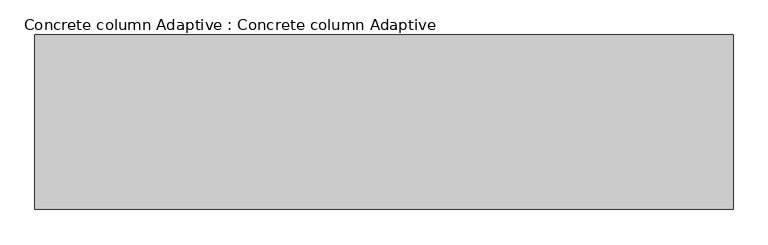
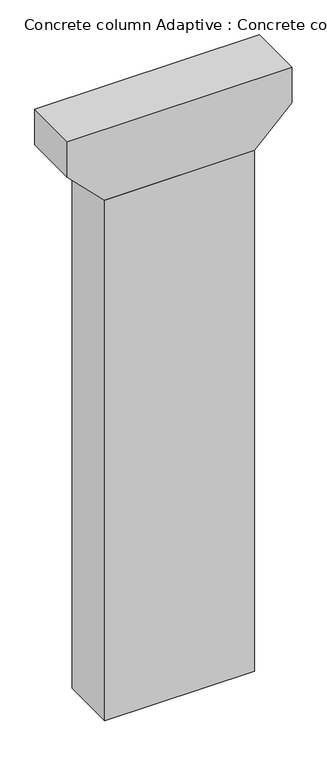
"""IFC4 building model written with IfcOpenShell, lengths in millimetres: proxy geometry, Concrete column Adaptive : Concrete column Adaptive."""

import ifcopenshell
import ifcopenshell.guid

model = None  # the IFC model being written
_history = None  # IfcOwnerHistory: only IFC2X3 demands one
_inside = {}  # id of a spatial element -> (the spatial element, [elements in it])
_under = {}  # id of a project, library or spatial element -> (it, [spatial elements below it])
_declared = {}  # id of a project -> (the project, [libraries it declares])
_typed = {}  # id of a type object -> (the type object, [elements of that type])
_made_of = {}  # id of a material, layer set ... -> (it, [elements and type objects made of it])


def new_model(schema):
    """Start an empty IFC model of exactly this schema.

    Asked for "IFC4X3", IfcOpenShell would pick the latest addendum, in which some entities
    have other attributes; the version numbers below select the first issue.
    IFC2X3 requires an IfcOwnerHistory on every rooted entity: one is made here for all.
    """
    global model, _history
    if schema == "IFC4X3":
        model = ifcopenshell.file(schema_version=(4, 3, 0, 0))
    else:
        model = ifcopenshell.file(schema=schema)
    _inside.clear()
    _under.clear()
    _declared.clear()
    _typed.clear()
    _made_of.clear()
    _history = None
    if model.schema == "IFC2X3":
        org = make("IfcOrganization", Name="unknown")
        user = make(
            "IfcPersonAndOrganization",
            ThePerson=make("IfcPerson", FamilyName="unknown"),
            TheOrganization=org,
        )
        app = make(
            "IfcApplication",
            ApplicationDeveloper=org,
            Version="unknown",
            ApplicationFullName="unknown",
            ApplicationIdentifier="unknown",
        )
        _history = make(
            "IfcOwnerHistory",
            OwningUser=user,
            OwningApplication=app,
            ChangeAction="ADDED",
            CreationDate=0,
        )
    return model


def make(cls, **values):
    """One entity of the class cls with the attributes given. An attribute that is None is left unset."""
    return model.create_entity(
        cls, **{name: value for name, value in values.items() if value is not None}
    )


def rooted(cls, **values):
    """An entity with a GlobalId (a new one), such as an element, a storey or a relation."""
    return make(cls, GlobalId=ifcopenshell.guid.new(), OwnerHistory=_history, **values)


def si_unit(unit_type, name, prefix=None):
    """IfcSIUnit, for example si_unit("LENGTHUNIT", "METRE", prefix="MILLI")."""
    return make("IfcSIUnit", UnitType=unit_type, Prefix=prefix, Name=name)


def assignment(units):
    """IfcUnitAssignment: the units of a project."""
    return None if units is None else make("IfcUnitAssignment", Units=units)


def point(xyz):
    """IfcCartesianPoint."""
    return None if xyz is None else make("IfcCartesianPoint", Coordinates=xyz)


def direction(xyz):
    """IfcDirection."""
    return None if xyz is None else make("IfcDirection", DirectionRatios=xyz)


def frame(location, z_axis=None, x_axis=None):
    """IfcAxis2Placement3D, a coordinate frame: its origin and axes. An axis left out is left unset."""
    return make(
        "IfcAxis2Placement3D",
        Location=point(location),
        Axis=direction(z_axis),
        RefDirection=direction(x_axis),
    )


def origin():
    """The frame at (0, 0, 0) with its axes left unset."""
    return frame((0.0, 0.0, 0.0))


def origin_with_axes():
    """The frame at (0, 0, 0) with the z axis (0, 0, 1) and the x axis (1, 0, 0) written out."""
    return frame((0.0, 0.0, 0.0), z_axis=(0.0, 0.0, 1.0), x_axis=(1.0, 0.0, 0.0))


def place(relative_to, where):
    """IfcLocalPlacement: puts the frame where relative to a parent placement (None: the world)."""
    return make(
        "IfcLocalPlacement", PlacementRelTo=relative_to, RelativePlacement=where
    )


def context(
    kind, dimensions, precision=None, world=None, true_north=None, identifier=None
):
    """IfcGeometricRepresentationContext, for example the 3D "Model" context."""
    return make(
        "IfcGeometricRepresentationContext",
        ContextIdentifier=identifier,
        ContextType=kind,
        CoordinateSpaceDimension=dimensions,
        Precision=precision,
        WorldCoordinateSystem=world,
        TrueNorth=true_north,
    )


def project(units=None, contexts=None):
    """IfcProject with its units and contexts."""
    return rooted(
        "IfcProject",
        Name="project",
        RepresentationContexts=contexts,
        UnitsInContext=assignment(units),
    )


def spatial(cls, under=None, at=None, **own):
    """A site, building, storey or space (cls), placed at a placement, below another one or the project."""
    s = rooted(cls, ObjectPlacement=at, **own)
    if under is not None:
        _under.setdefault(under.id(), (under, []))[1].append(s)
    return s


def polyline(points):
    """IfcPolyline through the points."""
    return make("IfcPolyline", Points=[point(p) for p in points])


def outline(outer, holes=None, kind="AREA"):
    """IfcArbitraryClosedProfileDef: a profile drawn as a closed curve; with holes, ...WithVoids."""
    if holes is None:
        return make("IfcArbitraryClosedProfileDef", ProfileType=kind, OuterCurve=outer)
    return make(
        "IfcArbitraryProfileDefWithVoids",
        ProfileType=kind,
        OuterCurve=outer,
        InnerCurves=holes,
    )


def extrude(swept, where, along, depth):
    """IfcExtrudedAreaSolid: the profile swept, set in the frame where, extruded along a direction by depth."""
    return make(
        "IfcExtrudedAreaSolid",
        SweptArea=swept,
        Position=where,
        ExtrudedDirection=direction(along),
        Depth=depth,
    )


def shape(context_of_items, identifier, shape_type, items):
    """IfcShapeRepresentation: the items that make up one representation, for example the "Body"."""
    return make(
        "IfcShapeRepresentation",
        ContextOfItems=context_of_items,
        RepresentationIdentifier=identifier,
        RepresentationType=shape_type,
        Items=items,
    )


def source(mapping_origin, context_of_items, identifier, shape_type, items):
    """IfcRepresentationMap: a shape defined once, which mapped items show again and again."""
    return make(
        "IfcRepresentationMap",
        MappingOrigin=mapping_origin,
        MappedRepresentation=shape(context_of_items, identifier, shape_type, items),
    )


def transform(
    local_origin,
    x_axis=None,
    y_axis=None,
    z_axis=None,
    scale=None,
    scale2=None,
    scale3=None,
    uniform=True,
):
    """IfcCartesianTransformationOperator3D, or its non-uniform kind. x_axis, y_axis, z_axis: its Axis1, 2, 3."""
    if uniform:
        return make(
            "IfcCartesianTransformationOperator3D",
            Axis1=direction(x_axis),
            Axis2=direction(y_axis),
            LocalOrigin=point(local_origin),
            Scale=scale,
            Axis3=direction(z_axis),
        )
    return make(
        "IfcCartesianTransformationOperator3DnonUniform",
        Axis1=direction(x_axis),
        Axis2=direction(y_axis),
        LocalOrigin=point(local_origin),
        Scale=scale,
        Axis3=direction(z_axis),
        Scale2=scale2,
        Scale3=scale3,
    )


def mapped(mapping_source, mapping_target):
    """IfcMappedItem: shows the shape of a source again, moved by a transform."""
    return make(
        "IfcMappedItem", MappingSource=mapping_source, MappingTarget=mapping_target
    )


def made_of(thing, what):
    """Note that an element or type object is made of a material, layer set ...; save() writes the relation."""
    if what is not None:
        _made_of.setdefault(what.id(), (what, []))[1].append(thing)
    return thing


def element(
    cls,
    number,
    at=None,
    inside=None,
    cuts=None,
    type_object=None,
    material=None,
    context=None,
    identifier="Body",
    shape_type=None,
    held_by="IfcProductDefinitionShape",
    body=None,
    shapes=None,
    **own,
):
    """One element of the class cls, such as IfcWall. Its Tag is "e" and its number.

    at: its placement. inside: the storey or other place that contains it. cuts: it is an
    opening in that element (IfcRelVoidsElement). A single representation is given by context,
    identifier, shape_type and body (its items); several are given by shapes. held_by: the class
    of the entity that holds the representations. save() writes the other relations.
    """
    e = rooted(cls, Tag="e%d" % number, ObjectPlacement=at, **own)
    if body is not None:
        shapes = [shape(context, identifier, shape_type, body)]
    if shapes is not None:
        e.Representation = make(held_by, Representations=shapes)
    if inside is not None:
        _inside.setdefault(inside.id(), (inside, []))[1].append(e)
    if cuts is not None:
        rooted(
            "IfcRelVoidsElement", RelatingBuildingElement=cuts, RelatedOpeningElement=e
        )
    if type_object is not None:
        _typed.setdefault(type_object.id(), (type_object, []))[1].append(e)
    return made_of(e, material)


def aggregate(whole, parts):
    """IfcRelAggregates: a whole, such as a stair, and the parts it consists of."""
    return rooted("IfcRelAggregates", RelatingObject=whole, RelatedObjects=parts)


def save(model, path):
    """Write the relations noted so far, then the file.

    IfcRelAggregates (storeys below a building ...), IfcRelContainedInSpatialStructure (elements
    in a storey), IfcRelDefinesByType, IfcRelAssociatesMaterial and IfcRelDeclares: one each for
    every whole, place, type object, material and project.
    """
    for whole, parts in _under.values():
        aggregate(whole, parts)
    for where, things in _inside.values():
        rooted(
            "IfcRelContainedInSpatialStructure",
            RelatedElements=things,
            RelatingStructure=where,
        )
    for kind, things in _typed.values():
        rooted("IfcRelDefinesByType", RelatedObjects=things, RelatingType=kind)
    for what, things in _made_of.values():
        rooted("IfcRelAssociatesMaterial", RelatedObjects=things, RelatingMaterial=what)
    for by, libraries in _declared.values():
        rooted("IfcRelDeclares", RelatingContext=by, RelatedDefinitions=libraries)
    model.write(path)


def concrete_column_adaptive_concrete_column_adaptive_c5f28f15(model_context):
    return source(origin(), model_context, "Body", "SweptSolid", [
        extrude(outline(polyline([(33382.0, 6000.0), (33382.0, -6000.0), (31382.0, -6000.0), (29382.0, -4000.0), (29382.0, 4000.0), (31382.0, 6000.0), (33382.0, 6000.0)])), frame((0.0, -1500.0, 0.0), z_axis=(0.0, 1.0, 0.0), x_axis=(0.0, 0.0, 1.0)), (0.0, 0.0, 1.0), 3000.0),
        extrude(outline(polyline([(-4000.0, -1500.0), (-4000.0, 1500.0), (4000.0, 1500.0), (4000.0, -1500.0), (-4000.0, -1500.0)])), origin_with_axes(), (0.0, 0.0, 1.0), 29382.0),
    ])


if __name__ == "__main__":
    model = new_model("IFC4")
    model_context = context("Model", 3, world=origin())
    ifc_project = project(units=[si_unit("LENGTHUNIT", "METRE", prefix="MILLI")], contexts=[model_context])
    site = spatial("IfcSite", under=ifc_project)
    building = spatial("IfcBuilding", under=site)
    placement = place(None, origin())
    concrete_column_adaptive_concrete_column_adaptive_shape = concrete_column_adaptive_concrete_column_adaptive_c5f28f15(model_context)
    element("IfcBuildingElementProxy", 1, Name="Concrete column Adaptive : Concrete column Adaptive", ObjectType="Concrete column Adaptive : Concrete column Adaptive", at=placement, inside=building, context=model_context, shape_type="MappedRepresentation", body=[
        mapped(concrete_column_adaptive_concrete_column_adaptive_shape, transform((0.0, 0.0, 0.0), x_axis=(1.0, 0.0, 0.0), y_axis=(0.0, 1.0, 0.0), z_axis=(0.0, 0.0, 1.0))),
    ])
    save(model, "model.ifc")

# Revit data of these elements
# Type "Concrete column Adaptive : Concrete column Adaptive"
#   Height [instance default] = 30000 mm
#   Default Elevation = 0
# Element 1 (IfcBuildingElementProxy, "Concrete column Adaptive : Concrete column Adaptive")
#   Height = 29382 mm
